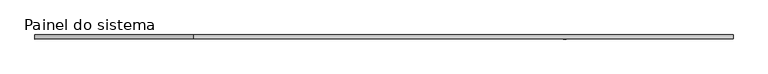
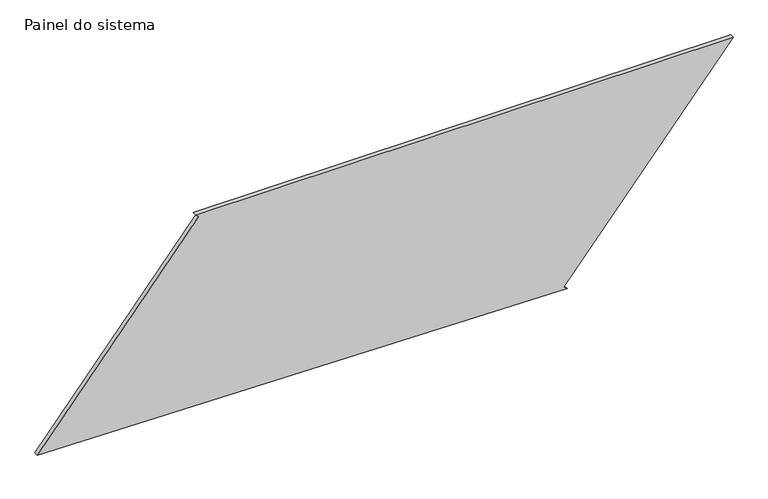
"""IFC4 building model written with IfcOpenShell, lengths in millimetres: plate geometry, Painel do sistema : Envidraçado."""

from ifc_helpers import new_model, si_unit, frame, origin, place, context, project, spatial, polyline, outline, extrude, source, transform, mapped, element, save


def painel_do_sistema_d31862cb(model_context):
    return source(origin(), model_context, "Body", "SweptSolid", [
        extrude(outline(polyline([(0.0, 1117.1651257), (15.8992441, 1097.8722763), (1277.1619897, 2137.2793579), (1277.1619897, -1163.9812392), (1261.2627456, -1144.6883899), (56.8087527, -2137.2793579), (0.0, 1117.1651257)])), frame((0.0, 24.5, 0.0), z_axis=(0.0, 1.0, 0.0), x_axis=(0.0, 0.0, 1.0)), (0.0, 0.0, 1.0), 25.0),
    ])


if __name__ == "__main__":
    model = new_model("IFC4")
    model_context = context("Model", 3, world=origin())
    ifc_project = project(units=[si_unit("LENGTHUNIT", "METRE", prefix="MILLI")], contexts=[model_context])
    site = spatial("IfcSite", under=ifc_project)
    building = spatial("IfcBuilding", under=site)
    placement = place(None, origin())
    painel_do_sistema_shape = painel_do_sistema_d31862cb(model_context)
    element("IfcPlate", 1, ObjectType="Painel do sistema : Envidraçado", at=placement, inside=building, context=model_context, shape_type="MappedRepresentation", body=[
        mapped(painel_do_sistema_shape, transform((0.0, 0.0, 0.0), x_axis=(1.0, 0.0, 0.0), y_axis=(0.0, 1.0, 0.0), z_axis=(0.0, 0.0, 1.0))),
    ])
    save(model, "model.ifc")

# Revit data of these elements
# Type "Painel do sistema : Envidraçado"
#   Construction Type Id = "GSP4R"
#   Analytic Construction = "Vidraça única Pilkington 1/8 pol"
#   Visual Light Transmittance = 0.9
#   Solar Heat Gain Coefficient = 0.86
#   Heat Transfer Coefficient (U) = 6.7069 W/(m²·K)
# Element 1 (IfcPlate, "Painel do sistema : Envidraçado")
#   Materials on its faces: "Vidro"
# Materials
#   "Vidro": class "Vidro", colour RGB 0 128 192, transparency 0.9, Description = "Vidro de sílica", Cost = 0
